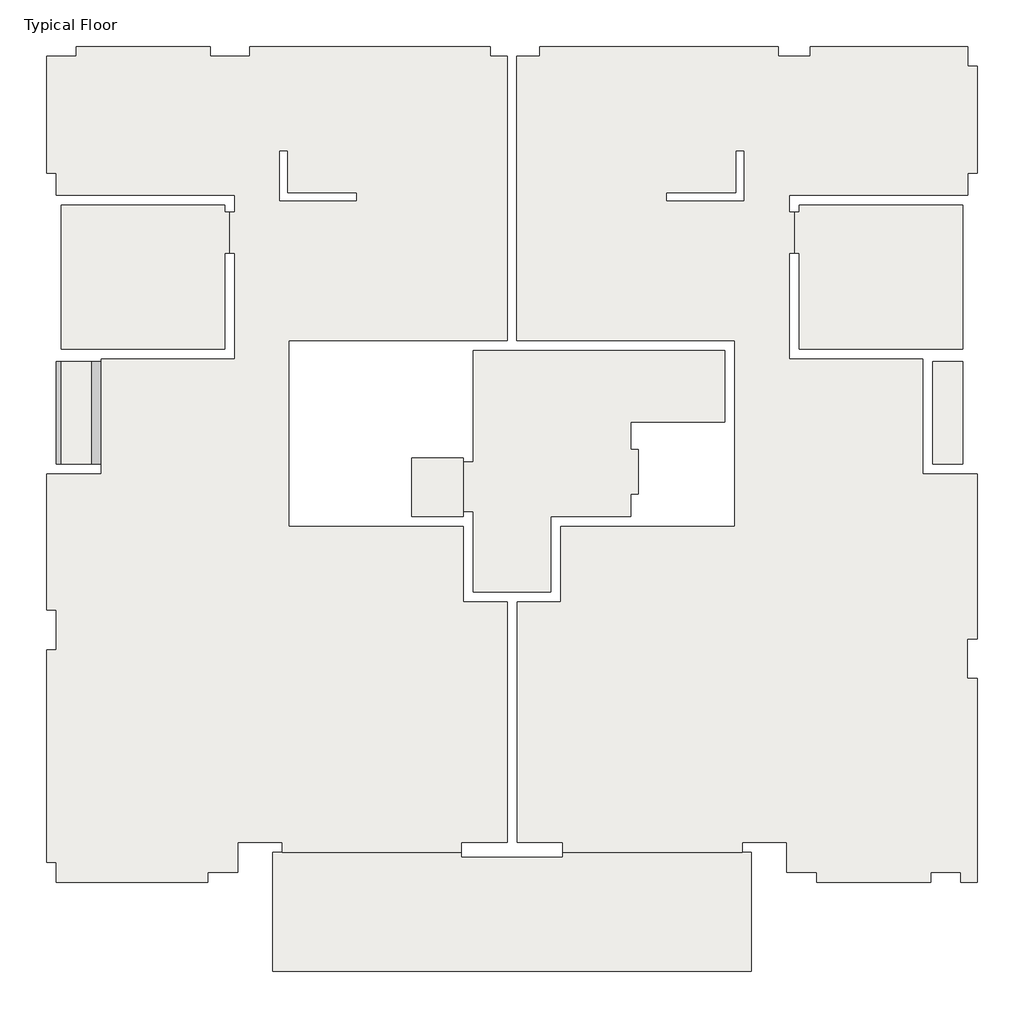
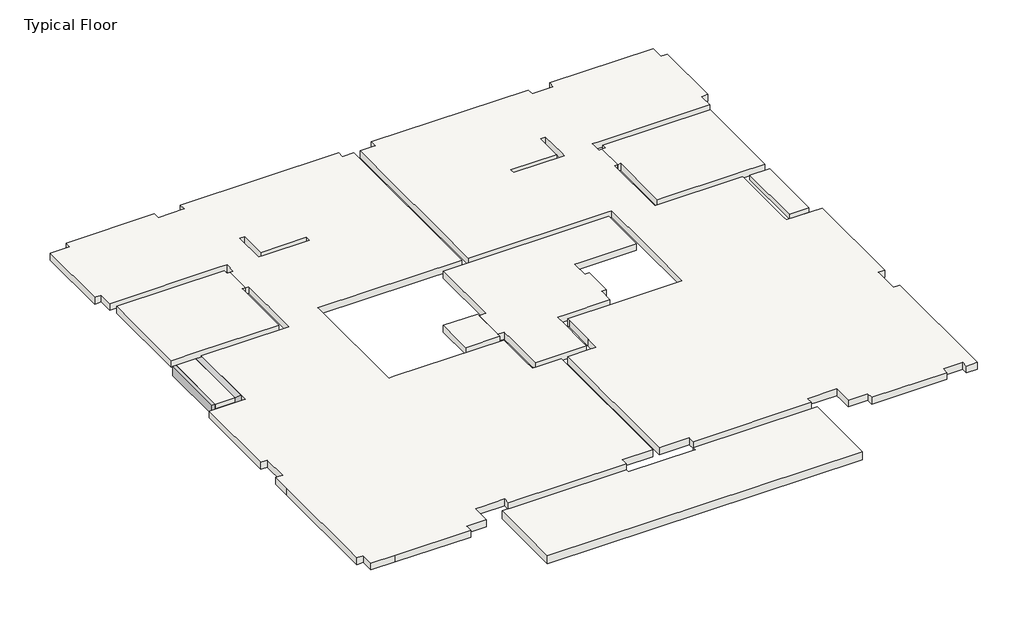
# One storey: 9 slabs, 2 beams.
"""IFC4 building model written with IfcOpenShell, lengths in millimetres."""

from ifc_helpers import new_model, si_unit, frame, origin, place, context, project, spatial, polyline, outline, extrude, faceted_brep, element, save

model = new_model("IFC4")

# Units and contexts
model_context = context("Model", 3, world=origin())
ifc_project = project(units=[si_unit("LENGTHUNIT", "METRE", prefix="MILLI")], contexts=[model_context])

# Site, building, storey
site = spatial("IfcSite", under=ifc_project)
building = spatial("IfcBuilding", under=site)
storey = spatial("IfcBuildingStorey", under=building, Name="Typical Floor", Elevation=3000.0)

# Beams
placement = place(None, origin())
element("IfcBeam", 1, ObjectType="Concrete Rectengular Beam : 10/30", at=placement, inside=storey, context=model_context, shape_type="Brep", body=[
    faceted_brep([(-47605.2156022, 29710.9648817, 3000.0), (-47505.2156022, 29710.9648817, 3000.0), (-47505.2156022, 31780.84273, 3000.0), (-47605.2156022, 31780.84273, 3000.0), (-47605.2156022, 29710.9648817, 2700.0), (-47605.2156022, 31780.84273, 2700.0), (-47505.2156022, 29710.9648817, 2700.0), (-47505.2156022, 31780.84273, 2700.0), (-47505.2156022, 29710.9648817, 2850.0), (-47505.2156022, 31780.84273, 2850.0)], [[[0, 1, 2, 3]], [[4, 0, 3, 5]], [[6, 4, 5, 7]], [[1, 8, 6, 7, 9, 2]], [[1, 0, 4, 6, 8]], [[3, 2, 9, 7, 5]]]),
])
element("IfcBeam", 2, ObjectType="Concrete Rectengular Beam : 20/50", at=placement, inside=storey, context=model_context, shape_type="Brep", body=[
    faceted_brep([(-46905.7952795, 29710.9648817, 3000.0), (-46705.7952795, 29710.9648817, 3000.0), (-46705.7952795, 31780.84273, 3000.0), (-46905.7952795, 31780.84273, 3000.0), (-46905.7952795, 29710.9648817, 2500.0), (-46905.7952795, 29710.9648817, 2850.0), (-46905.7952795, 31780.84273, 2850.0), (-46905.7952795, 31780.84273, 2500.0), (-46705.7952795, 29710.9648817, 2500.0), (-46705.7952795, 31780.84273, 2500.0), (-46705.7952795, 29710.9648817, 2780.0), (-46705.7952795, 31780.84273, 2780.0)], [[[0, 1, 2, 3]], [[4, 5, 0, 3, 6, 7]], [[8, 4, 7, 9]], [[2, 1, 10, 8, 9, 11]], [[1, 0, 5, 4, 8, 10]], [[3, 2, 11, 9, 7, 6]]]),
])

# Slabs
element("IfcSlab", 3, ObjectType="15", at=placement, inside=storey, context=model_context, shape_type="SweptSolid", body=[
    extrude(outline(polyline([(-29340.5251854, 31780.84273), (-29340.5251854, 29710.9648817), (-29944.302346, 29710.9648817), (-29944.302346, 31780.84273), (-29340.5251854, 31780.84273)])), frame((0.0, 0.0, 2850.0), z_axis=(0.0, 0.0, 1.0), x_axis=(1.0, 0.0, 0.0)), (0.0, 0.0, 1.0), 150.0),
])
element("IfcSlab", 4, ObjectType="15", at=placement, inside=storey, context=model_context, shape_type="SweptSolid", body=[
    extrude(outline(polyline([(-47505.2156022, 31780.84273), (-46905.7952795, 31780.84273), (-46905.7952795, 29710.9648817), (-47505.2156022, 29710.9648817), (-47505.2156022, 31780.84273)])), frame((0.0, 0.0, 2850.0), z_axis=(0.0, 0.0, 1.0), x_axis=(1.0, 0.0, 0.0)), (0.0, 0.0, 1.0), 150.0),
])
element("IfcSlab", 5, ObjectType="22", at=placement, inside=storey, context=model_context, shape_type="Brep", body=[
    faceted_brep([(-29045.7952795, 21280.2897882, 2780.0), (-29382.308052, 21280.2897882, 2780.0), (-29382.308052, 21480.2897882, 2780.0), (-29982.308052, 21480.2897882, 2780.0), (-29982.308052, 21280.2897882, 2780.0), (-32286.4740574, 21280.2897882, 2780.0), (-32286.4740574, 21480.2897882, 2780.0), (-32886.4740574, 21480.2897882, 2780.0), (-32886.4740574, 21880.2897882, 2780.0), (-32886.4740574, 22080.2897882, 2780.0), (-33786.4740574, 22080.2897882, 2780.0), (-33786.4740574, 21880.2897882, 2780.0), (-37400.2620822, 21880.2897882, 2780.0), (-37400.2620822, 22079.8085502, 2780.0), (-38324.2014504, 22079.8085502, 2780.0), (-38324.2014504, 26934.5299537, 2780.0), (-37644.7021495, 26934.5299537, 2780.0), (-37444.7021495, 26934.5299537, 2780.0), (-37444.7021495, 27352.982888, 2780.0), (-37444.7021495, 28354.1914622, 2780.0), (-37444.7021495, 28454.7268324, 2780.0), (-35957.8992549, 28454.7268324, 2780.0), (-33933.139307, 28454.7268324, 2780.0), (-33933.139307, 28754.7268324, 2780.0), (-33933.139307, 30454.4375606, 2780.0), (-33933.139307, 32204.3938202, 2780.0), (-34133.139307, 32204.3938202, 2780.0), (-38325.2180585, 32204.3938202, 2780.0), (-38325.2180585, 37931.0505674, 2780.0), (-37865.9301848, 37931.0505674, 2780.0), (-37865.9301848, 38131.0505674, 2780.0), (-33061.2774622, 38131.0505674, 2780.0), (-33061.2774622, 37931.0505674, 2780.0), (-32411.2774622, 37931.0505674, 2780.0), (-32411.2774622, 38131.0505674, 2780.0), (-29244.7343642, 38131.0505674, 2780.0), (-29244.7343642, 37731.0505674, 2780.0), (-29044.7343642, 37731.0505674, 2780.0), (-29044.7343642, 35580.4654108, 2780.0), (-29244.7343642, 35580.4654108, 2780.0), (-29244.7343642, 35129.640202, 2780.0), (-32634.5879334, 35129.640202, 2780.0), (-32834.5879334, 35129.640202, 2780.0), (-32834.5879334, 34793.0831223, 2780.0), (-32734.5879334, 34793.0831223, 2780.0), (-32734.5879334, 33965.4699454, 2780.0), (-32834.5879334, 33965.4699454, 2780.0), (-32834.5879334, 32030.84273, 2780.0), (-32834.5879334, 31830.84273, 2780.0), (-30144.302346, 31830.84273, 2780.0), (-30144.302346, 31780.84273, 2780.0), (-30144.302346, 29710.9648817, 2780.0), (-30144.302346, 29510.9648817, 2780.0), (-29045.7952795, 29510.9648817, 2780.0), (-29045.7952795, 26190.9393744, 2780.0), (-29245.7952795, 26190.9393744, 2780.0), (-29245.7952795, 25390.9393744, 2780.0), (-29045.7952795, 25390.9393744, 2780.0), (-33753.2522949, 36022.8722618, 2780.0), (-33903.2522949, 36022.8722618, 2780.0), (-33903.2522949, 35173.7904306, 2780.0), (-35302.6288773, 35173.7904306, 2780.0), (-35302.6288773, 35023.7904306, 2780.0), (-33753.2522949, 35023.7904306, 2780.0), (-33753.2522949, 35173.7904306, 2780.0), (-29382.308052, 21280.2897882, 3000.0), (-29045.7952795, 21280.2897882, 3000.0), (-29045.7952795, 25390.9393744, 3000.0), (-29245.7952795, 25390.9393744, 3000.0), (-29245.7952795, 26190.9393744, 3000.0), (-29045.7952795, 26190.9393744, 3000.0), (-29045.7952795, 29510.9648817, 3000.0), (-30144.302346, 29510.9648817, 3000.0), (-30144.302346, 29710.9648817, 3000.0), (-30144.302346, 31780.84273, 3000.0), (-30144.302346, 31830.84273, 3000.0), (-32834.5879334, 31830.84273, 3000.0), (-32834.5879334, 32030.84273, 3000.0), (-32834.5879334, 33965.4699454, 3000.0), (-32734.5879334, 33965.4699454, 3000.0), (-32734.5879334, 34793.0831223, 3000.0), (-32834.5879334, 34793.0831223, 3000.0), (-32834.5879334, 35129.640202, 3000.0), (-32634.5879334, 35129.640202, 3000.0), (-29244.7343642, 35129.640202, 3000.0), (-29244.7343642, 35580.4654108, 3000.0), (-29044.7343642, 35580.4654108, 3000.0), (-29044.7343642, 37731.0505674, 3000.0), (-29244.7343642, 37731.0505674, 3000.0), (-29244.7343642, 38131.0505674, 3000.0), (-32411.2774622, 38131.0505674, 3000.0), (-32411.2774622, 37931.0505674, 3000.0), (-33061.2774622, 37931.0505674, 3000.0), (-33061.2774622, 38131.0505674, 3000.0), (-37865.9301848, 38131.0505674, 3000.0), (-37865.9301848, 37931.0505674, 3000.0), (-38325.2180585, 37931.0505674, 3000.0), (-38325.2180585, 32204.3938202, 3000.0), (-34133.139307, 32204.3938202, 3000.0), (-33933.139307, 32204.3938202, 3000.0), (-33933.139307, 30454.4375606, 3000.0), (-33933.139307, 28754.7268324, 3000.0), (-33933.139307, 28454.7268324, 3000.0), (-35957.8992549, 28454.7268324, 3000.0), (-37444.7021495, 28454.7268324, 3000.0), (-37444.7021495, 28354.1914622, 3000.0), (-37444.7021495, 27352.982888, 3000.0), (-37444.7021495, 26934.5299537, 3000.0), (-37644.7021495, 26934.5299537, 3000.0), (-38324.2014504, 26934.5299537, 3000.0), (-38324.2014504, 22079.8085502, 3000.0), (-37400.2620822, 22079.8085502, 3000.0), (-37400.2620822, 21880.2897882, 3000.0), (-33786.4740574, 21880.2897882, 3000.0), (-33786.4740574, 22080.2897882, 3000.0), (-32886.4740574, 22080.2897882, 3000.0), (-32886.4740574, 21880.2897882, 3000.0), (-32886.4740574, 21480.2897882, 3000.0), (-32286.4740574, 21480.2897882, 3000.0), (-32286.4740574, 21280.2897882, 3000.0), (-29982.308052, 21280.2897882, 3000.0), (-29982.308052, 21480.2897882, 3000.0), (-29382.308052, 21480.2897882, 3000.0), (-33903.2522949, 36022.8722618, 3000.0), (-33753.2522949, 36022.8722618, 3000.0), (-33753.2522949, 35173.7904306, 3000.0), (-33753.2522949, 35023.7904306, 3000.0), (-35302.6288773, 35023.7904306, 3000.0), (-35302.6288773, 35173.7904306, 3000.0), (-33903.2522949, 35173.7904306, 3000.0), (-37400.2620822, 21880.2897882, 2800.0)], [[[0, 1, 2, 3, 4, 5, 6, 7, 8, 9, 10, 11, 12, 13, 14, 15, 16, 17, 18, 19, 20, 21, 22, 23, 24, 25, 26, 27, 28, 29, 30, 31, 32, 33, 34, 35, 36, 37, 38, 39, 40, 41, 42, 43, 44, 45, 46, 47, 48, 49, 50, 51, 52, 53, 54, 55, 56, 57], [58, 59, 60, 61, 62, 63, 64]], [[65, 66, 67, 68, 69, 70, 71, 72, 73, 74, 75, 76, 77, 78, 79, 80, 81, 82, 83, 84, 85, 86, 87, 88, 89, 90, 91, 92, 93, 94, 95, 96, 97, 98, 99, 100, 101, 102, 103, 104, 105, 106, 107, 108, 109, 110, 111, 112, 113, 114, 115, 116, 117, 118, 119, 120, 121, 122], [123, 124, 125, 126, 127, 128, 129]], [[1, 0, 66, 65]], [[2, 1, 65, 122]], [[3, 2, 122, 121]], [[4, 3, 121, 120]], [[5, 4, 120, 119]], [[6, 5, 119, 118]], [[7, 6, 118, 117]], [[7, 117, 116, 115, 9, 8]], [[10, 9, 115, 114]], [[11, 10, 114, 113]], [[12, 11, 113, 112, 130]], [[13, 12, 130, 112, 111]], [[14, 13, 111, 110]], [[15, 14, 110, 109]], [[15, 109, 108, 107, 17, 16]], [[18, 17, 107, 106]], [[19, 18, 106, 105]], [[20, 19, 105, 104]], [[20, 104, 103, 102, 22, 21]], [[22, 102, 101, 100, 99, 25, 24, 23]], [[25, 99, 98, 97, 27, 26]], [[28, 27, 97, 96]], [[29, 28, 96, 95]], [[30, 29, 95, 94]], [[31, 30, 94, 93]], [[32, 31, 93, 92]], [[33, 32, 92, 91]], [[34, 33, 91, 90]], [[35, 34, 90, 89]], [[38, 37, 87, 86]], [[39, 38, 86, 85]], [[40, 39, 85, 84]], [[40, 84, 83, 82, 42, 41]], [[43, 42, 82, 81]], [[44, 43, 81, 80]], [[45, 44, 80, 79]], [[46, 45, 79, 78]], [[46, 78, 77, 76, 48, 47]], [[49, 48, 76, 75]], [[49, 75, 74, 73, 72, 52, 51, 50]], [[53, 52, 72, 71]], [[53, 71, 70, 54]], [[0, 57, 67, 66]], [[59, 58, 124, 123]], [[60, 59, 123, 129]], [[61, 60, 129, 128]], [[62, 61, 128, 127]], [[63, 62, 127, 126]], [[63, 126, 125, 124, 58, 64]], [[56, 68, 67, 57]], [[68, 56, 55, 69]], [[69, 55, 54, 70]], [[36, 35, 89, 88]], [[37, 36, 88, 87]]]),
])
element("IfcSlab", 6, ObjectType="22", at=placement, inside=storey, context=model_context, shape_type="Brep", body=[
    faceted_brep([(-44556.7079689, 21280.2897882, 2780.0), (-46866.0948487, 21280.2897882, 2780.0), (-47605.7952795, 21280.2897882, 2780.0), (-47605.7952795, 21680.2897882, 2780.0), (-47805.7952795, 21680.2897882, 2780.0), (-47805.7952795, 25390.9393744, 2780.0), (-47805.7952795, 25968.694731, 2780.0), (-47605.7952795, 25968.694731, 2780.0), (-47605.7952795, 26768.694731, 2780.0), (-47805.7952795, 26768.694731, 2780.0), (-47805.7952795, 29510.9648817, 2780.0), (-46705.7952795, 29510.9648817, 2780.0), (-46705.7952795, 29710.9648817, 2780.0), (-46705.7952795, 31780.84273, 2780.0), (-46705.7952795, 31830.84273, 2780.0), (-44015.8481835, 31830.84273, 2780.0), (-44015.8481835, 32030.84273, 2780.0), (-44015.8481835, 33965.4699454, 2780.0), (-44113.8149674, 33965.4699454, 2780.0), (-44113.8149674, 34793.0831223, 2780.0), (-44015.8481835, 34793.0831223, 2780.0), (-44015.8481835, 35129.640202, 2780.0), (-44215.8481835, 35129.640202, 2780.0), (-47605.7017527, 35129.640202, 2780.0), (-47605.7017527, 35580.4654108, 2780.0), (-47805.7017527, 35580.4654108, 2780.0), (-47805.7017527, 37931.0505674, 2780.0), (-47205.7952795, 37931.0505674, 2780.0), (-47205.7952795, 38131.0505674, 2780.0), (-44508.0144156, 38131.0505674, 2780.0), (-44508.0144156, 37931.0505674, 2780.0), (-43708.0144156, 37931.0505674, 2780.0), (-43708.0144156, 38131.0505674, 2780.0), (-38865.9301848, 38131.0505674, 2780.0), (-38865.9301848, 37931.0505674, 2780.0), (-38525.2180585, 37931.0505674, 2780.0), (-38525.2180585, 32204.3938202, 2780.0), (-42920.5336878, 32204.3938202, 2780.0), (-42920.5336878, 32004.3938202, 2780.0), (-42920.5336878, 28453.6610046, 2780.0), (-42720.5336878, 28453.6610046, 2780.0), (-39404.7173594, 28453.6610046, 2780.0), (-39404.7173594, 28354.1914622, 2780.0), (-39404.7173594, 27352.982888, 2780.0), (-39404.7173594, 26934.5299537, 2780.0), (-39204.7173594, 26934.5299537, 2780.0), (-38524.2014504, 26934.5299537, 2780.0), (-38524.2014504, 22079.8085502, 2780.0), (-39449.2017338, 22079.8085502, 2780.0), (-39449.2017338, 21880.2897882, 2780.0), (-43056.7079689, 21880.2897882, 2780.0), (-43056.7079689, 22080.2897882, 2780.0), (-43756.7079689, 22080.2897882, 2780.0), (-43956.7079689, 22080.2897882, 2780.0), (-43956.7079689, 21480.2897882, 2780.0), (-44556.7079689, 21480.2897882, 2780.0), (-42958.8833647, 36022.8722618, 2780.0), (-43108.8833647, 36022.8722618, 2780.0), (-43108.8833647, 35023.7904306, 2780.0), (-42958.8833647, 35023.7904306, 2780.0), (-41563.7602683, 35023.7904306, 2780.0), (-41563.7602683, 35173.7904306, 2780.0), (-42958.8833647, 35173.7904306, 2780.0), (-46866.0948487, 21280.2897882, 3000.0), (-44556.7079689, 21280.2897882, 3000.0), (-44556.7079689, 21480.2897882, 3000.0), (-43956.7079689, 21480.2897882, 3000.0), (-43956.7079689, 22080.2897882, 3000.0), (-43756.7079689, 22080.2897882, 3000.0), (-43056.7079689, 22080.2897882, 3000.0), (-43056.7079689, 21880.2897882, 3000.0), (-39449.2017338, 21880.2897882, 3000.0), (-39449.2017338, 22079.8085502, 3000.0), (-38524.2014504, 22079.8085502, 3000.0), (-38524.2014504, 26934.5299537, 3000.0), (-39204.7173594, 26934.5299537, 3000.0), (-39404.7173594, 26934.5299537, 3000.0), (-39404.7173594, 27352.982888, 3000.0), (-39404.7173594, 28354.1914622, 3000.0), (-39404.7173594, 28453.6610046, 3000.0), (-42720.5336878, 28453.6610046, 3000.0), (-42920.5336878, 28453.6610046, 3000.0), (-42920.5336878, 32004.3938202, 3000.0), (-42920.5336878, 32204.3938202, 3000.0), (-38525.2180585, 32204.3938202, 3000.0), (-38525.2180585, 37931.0505674, 3000.0), (-38865.9301848, 37931.0505674, 3000.0), (-38865.9301848, 38131.0505674, 3000.0), (-43708.0144156, 38131.0505674, 3000.0), (-43708.0144156, 37931.0505674, 3000.0), (-44508.0144156, 37931.0505674, 3000.0), (-44508.0144156, 38131.0505674, 3000.0), (-47205.7952795, 38131.0505674, 3000.0), (-47205.7952795, 37931.0505674, 3000.0), (-47805.7017527, 37931.0505674, 3000.0), (-47805.7017527, 35580.4654108, 3000.0), (-47605.7017527, 35580.4654108, 3000.0), (-47605.7017527, 35129.640202, 3000.0), (-44215.8481835, 35129.640202, 3000.0), (-44015.8481835, 35129.640202, 3000.0), (-44015.8481835, 34793.0831223, 3000.0), (-44113.8149674, 34793.0831223, 3000.0), (-44113.8149674, 33965.4699454, 3000.0), (-44015.8481835, 33965.4699454, 3000.0), (-44015.8481835, 32030.84273, 3000.0), (-44015.8481835, 31830.84273, 3000.0), (-46705.7952795, 31830.84273, 3000.0), (-46705.7952795, 31780.84273, 3000.0), (-46705.7952795, 29710.9648817, 3000.0), (-46705.7952795, 29510.9648817, 3000.0), (-47805.7952795, 29510.9648817, 3000.0), (-47805.7952795, 26768.694731, 3000.0), (-47605.7952795, 26768.694731, 3000.0), (-47605.7952795, 25968.694731, 3000.0), (-47805.7952795, 25968.694731, 3000.0), (-47805.7952795, 25390.9393744, 3000.0), (-47805.7952795, 21680.2897882, 3000.0), (-47605.7952795, 21680.2897882, 3000.0), (-47605.7952795, 21280.2897882, 3000.0), (-43108.8833647, 36022.8722618, 3000.0), (-42958.8833647, 36022.8722618, 3000.0), (-42958.8833647, 35173.7904306, 3000.0), (-41563.7602683, 35173.7904306, 3000.0), (-41563.7602683, 35023.7904306, 3000.0), (-42958.8833647, 35023.7904306, 3000.0), (-43108.8833647, 35023.7904306, 3000.0), (-39449.2017338, 21880.2897882, 2800.0)], [[[0, 1, 2, 3, 4, 5, 6, 7, 8, 9, 10, 11, 12, 13, 14, 15, 16, 17, 18, 19, 20, 21, 22, 23, 24, 25, 26, 27, 28, 29, 30, 31, 32, 33, 34, 35, 36, 37, 38, 39, 40, 41, 42, 43, 44, 45, 46, 47, 48, 49, 50, 51, 52, 53, 54, 55], [56, 57, 58, 59, 60, 61, 62]], [[63, 64, 65, 66, 67, 68, 69, 70, 71, 72, 73, 74, 75, 76, 77, 78, 79, 80, 81, 82, 83, 84, 85, 86, 87, 88, 89, 90, 91, 92, 93, 94, 95, 96, 97, 98, 99, 100, 101, 102, 103, 104, 105, 106, 107, 108, 109, 110, 111, 112, 113, 114, 115, 116, 117, 118], [119, 120, 121, 122, 123, 124, 125]], [[1, 0, 64, 63]], [[0, 55, 65, 64]], [[55, 54, 66, 65]], [[54, 53, 67, 66]], [[51, 69, 68, 67, 53, 52]], [[51, 50, 70, 69]], [[50, 49, 126, 71, 70]], [[49, 48, 72, 71, 126]], [[48, 47, 73, 72]], [[47, 46, 74, 73]], [[44, 76, 75, 74, 46, 45]], [[44, 43, 77, 76]], [[43, 42, 78, 77]], [[42, 41, 79, 78]], [[39, 81, 80, 79, 41, 40]], [[37, 83, 82, 81, 39, 38]], [[37, 36, 84, 83]], [[36, 35, 85, 84]], [[35, 34, 86, 85]], [[34, 33, 87, 86]], [[33, 32, 88, 87]], [[32, 31, 89, 88]], [[31, 30, 90, 89]], [[30, 29, 91, 90]], [[29, 28, 92, 91]], [[26, 25, 95, 94]], [[25, 24, 96, 95]], [[24, 23, 97, 96]], [[21, 99, 98, 97, 23, 22]], [[21, 20, 100, 99]], [[20, 19, 101, 100]], [[19, 18, 102, 101]], [[18, 17, 103, 102]], [[15, 105, 104, 103, 17, 16]], [[15, 14, 106, 105]], [[11, 109, 108, 107, 106, 14, 13, 12]], [[11, 10, 110, 109]], [[10, 9, 111, 110]], [[5, 4, 116, 115]], [[27, 26, 94, 93]], [[28, 27, 93, 92]], [[57, 56, 120, 119]], [[58, 57, 119, 125]], [[58, 125, 124, 123, 60, 59]], [[61, 60, 123, 122]], [[62, 61, 122, 121]], [[56, 62, 121, 120]], [[2, 1, 63, 118]], [[6, 5, 115, 114]], [[7, 6, 114, 113]], [[8, 7, 113, 112]], [[9, 8, 112, 111]], [[3, 2, 118, 117]], [[4, 3, 117, 116]]]),
])
element("IfcSlab", 7, ObjectType="22", at=placement, inside=storey, context=model_context, shape_type="Brep", body=[
    faceted_brep([(-37644.7021495, 27134.5299537, 2780.0), (-39204.7173594, 27134.5299537, 2780.0), (-39204.7173594, 27352.982888, 2780.0), (-39204.7173594, 28354.1914622, 2780.0), (-39204.7173594, 28754.2406819, 2780.0), (-39404.7173594, 28754.2406819, 2780.0), (-39404.7173594, 29753.278206, 2780.0), (-39204.7173594, 29753.278206, 2780.0), (-39204.7173594, 32004.3938202, 2780.0), (-34133.139307, 32004.3938202, 2780.0), (-34133.139307, 30554.4375606, 2780.0), (-35882.8992549, 30554.4375606, 2780.0), (-36032.8992549, 30554.4375606, 2780.0), (-36032.8992549, 30005.16433, 2780.0), (-35882.8992549, 30005.16433, 2780.0), (-35882.8992549, 29103.4696053, 2780.0), (-36032.8992549, 29103.4696053, 2780.0), (-36032.8992549, 28654.7268324, 2780.0), (-37444.7021495, 28654.7268324, 2780.0), (-37644.7021495, 28654.7268324, 2780.0), (-37644.7021495, 28354.1914622, 2780.0), (-37644.7021495, 27352.982888, 2780.0), (-39204.7173594, 27134.5299537, 3000.0), (-37644.7021495, 27134.5299537, 3000.0), (-37644.7021495, 27352.982888, 3000.0), (-37644.7021495, 28354.1914622, 3000.0), (-37644.7021495, 28654.7268324, 3000.0), (-37444.7021495, 28654.7268324, 3000.0), (-36032.8992549, 28654.7268324, 3000.0), (-36032.8992549, 29103.4696053, 3000.0), (-35882.8992549, 29103.4696053, 3000.0), (-35882.8992549, 30005.16433, 3000.0), (-36032.8992549, 30005.16433, 3000.0), (-36032.8992549, 30554.4375606, 3000.0), (-35882.8992549, 30554.4375606, 3000.0), (-34133.139307, 30554.4375606, 3000.0), (-34133.139307, 32004.3938202, 3000.0), (-39204.7173594, 32004.3938202, 3000.0), (-39204.7173594, 29753.278206, 3000.0), (-39404.7173594, 29753.278206, 3000.0), (-39404.7173594, 28754.2406819, 3000.0), (-39204.7173594, 28754.2406819, 3000.0), (-39204.7173594, 28354.1914622, 3000.0), (-39204.7173594, 27352.982888, 3000.0)], [[[0, 1, 2, 3, 4, 5, 6, 7, 8, 9, 10, 11, 12, 13, 14, 15, 16, 17, 18, 19, 20, 21]], [[22, 23, 24, 25, 26, 27, 28, 29, 30, 31, 32, 33, 34, 35, 36, 37, 38, 39, 40, 41, 42, 43]], [[1, 0, 23, 22]], [[1, 22, 43, 42, 41, 4, 3, 2]], [[5, 4, 41, 40]], [[6, 5, 40, 39]], [[7, 6, 39, 38]], [[8, 7, 38, 37]], [[9, 8, 37, 36]], [[10, 9, 36, 35]], [[10, 35, 34, 33, 12, 11]], [[13, 12, 33, 32]], [[14, 13, 32, 31]], [[15, 14, 31, 30]], [[16, 15, 30, 29]], [[17, 16, 29, 28]], [[17, 28, 27, 26, 19, 18]], [[19, 26, 25, 24, 23, 0, 21, 20]]]),
])
element("IfcSlab", 8, ObjectType="22", at=placement, inside=storey, context=model_context, shape_type="Brep", body=[
    faceted_brep([(-32634.5879334, 34793.0831223, 2780.0), (-32634.5879334, 34929.640202, 2780.0), (-29344.7343642, 34929.640202, 2780.0), (-29344.7343642, 32030.84273, 2780.0), (-32634.5879334, 32030.84273, 2780.0), (-32634.5879334, 33965.4699454, 2780.0), (-32734.5879334, 33965.4699454, 2780.0), (-32734.5879334, 34793.0831223, 2780.0), (-32634.5879334, 34929.640202, 3000.0), (-32634.5879334, 34793.0831223, 3000.0), (-32734.5879334, 34793.0831223, 3000.0), (-32734.5879334, 33965.4699454, 3000.0), (-32634.5879334, 33965.4699454, 3000.0), (-32634.5879334, 32030.84273, 3000.0), (-30144.302346, 32030.84273, 3000.0), (-29344.7343642, 32030.84273, 3000.0), (-29344.7343642, 34929.640202, 3000.0)], [[[0, 1, 2, 3, 4, 5, 6, 7]], [[8, 9, 10, 11, 12, 13, 14, 15, 16]], [[1, 0, 9, 8]], [[2, 1, 8, 16]], [[3, 2, 16, 15]], [[4, 3, 15, 14, 13]], [[5, 4, 13, 12]], [[6, 5, 12, 11]], [[7, 6, 11, 10]], [[0, 7, 10, 9]]]),
])
element("IfcSlab", 9, ObjectType="22", at=placement, inside=storey, context=model_context, shape_type="Brep", body=[
    faceted_brep([(-44215.8481835, 34929.640202, 2780.0), (-44215.8481835, 34793.0831223, 2780.0), (-44113.8149674, 34793.0831223, 2780.0), (-44113.8149674, 33965.4699454, 2780.0), (-44215.8481835, 33965.4699454, 2780.0), (-44215.8481835, 32030.84273, 2780.0), (-47505.7017527, 32030.84273, 2780.0), (-47505.7017527, 34929.640202, 2780.0), (-44215.8481835, 34793.0831223, 3000.0), (-44215.8481835, 34929.640202, 3000.0), (-47505.7017527, 34929.640202, 3000.0), (-47505.7017527, 32030.84273, 3000.0), (-46705.7952795, 32030.84273, 3000.0), (-44215.8481835, 32030.84273, 3000.0), (-44215.8481835, 33965.4699454, 3000.0), (-44113.8149674, 33965.4699454, 3000.0), (-44113.8149674, 34793.0831223, 3000.0)], [[[0, 1, 2, 3, 4, 5, 6, 7]], [[8, 9, 10, 11, 12, 13, 14, 15, 16]], [[1, 0, 9, 8]], [[2, 1, 8, 16]], [[3, 2, 16, 15]], [[4, 3, 15, 14]], [[4, 14, 13, 5]], [[10, 7, 6, 11]], [[0, 7, 10, 9]], [[5, 13, 12, 11, 6]]]),
])
element("IfcSlab", 10, ObjectType="22", at=placement, inside=storey, context=model_context, shape_type="Brep", body=[
    faceted_brep([(-40450.3660009, 29837.9491617, 2780.0), (-39404.7173594, 29837.9491617, 2780.0), (-39404.7173594, 29753.278206, 2780.0), (-39404.7173594, 28754.2406819, 2780.0), (-39404.7173594, 28653.6610046, 2780.0), (-40450.3660009, 28653.6610046, 2780.0), (-39404.7173594, 29837.9491617, 3000.0), (-40450.3660009, 29837.9491617, 3000.0), (-40450.3660009, 28653.6610046, 3000.0), (-39404.7173594, 28653.6610046, 3000.0), (-39404.7173594, 28754.2406819, 3000.0), (-39404.7173594, 29753.278206, 3000.0)], [[[0, 1, 2, 3, 4, 5]], [[6, 7, 8, 9, 10, 11]], [[1, 0, 7, 6]], [[3, 2, 1, 6, 11, 10]], [[3, 10, 9, 4]], [[7, 0, 5, 8]], [[5, 4, 9, 8]]]),
])
element("IfcSlab", 11, ObjectType="26", at=placement, inside=storey, context=model_context, shape_type="Brep", body=[
    faceted_brep([(-39449.2017338, 21880.2897882, 2540.0), (-39449.2017338, 21779.8085502, 2540.0), (-37400.2620822, 21779.8085502, 2540.0), (-37400.2620822, 21880.2897882, 2540.0), (-33605.0891993, 21880.2897882, 2540.0), (-33605.0891993, 19481.1095176, 2540.0), (-43243.3137014, 19481.1095176, 2540.0), (-43243.3137014, 21880.2897882, 2540.0), (-39449.2017338, 21779.8085502, 2800.0), (-39449.2017338, 21880.2897882, 2800.0), (-43056.7079689, 21880.2897882, 2800.0), (-43243.3137014, 21880.2897882, 2800.0), (-43243.3137014, 19481.1095176, 2800.0), (-33605.0891993, 19481.1095176, 2800.0), (-33605.0891993, 21880.2897882, 2800.0), (-33786.4740574, 21880.2897882, 2800.0), (-37400.2620822, 21880.2897882, 2800.0), (-37400.2620822, 21779.8085502, 2800.0), (-39449.2017338, 21880.2897882, 2780.0), (-37400.2620822, 21880.2897882, 2780.0), (-33605.0891993, 21880.2897882, 2600.0), (-33605.0891993, 19481.1095176, 2600.0), (-43243.3137014, 19481.1095176, 2600.0), (-43243.3137014, 21880.2897882, 2600.0)], [[[0, 1, 2, 3, 4, 5, 6, 7]], [[8, 9, 10, 11, 12, 13, 14, 15, 16, 17]], [[1, 0, 18, 9, 8]], [[2, 1, 8, 17]], [[3, 2, 17, 16, 19]], [[4, 3, 19, 16, 15, 14, 20]], [[5, 4, 20, 14, 13, 21]], [[6, 5, 21, 13, 12, 22]], [[7, 6, 22, 12, 11, 23]], [[0, 7, 23, 11, 10, 9, 18]]]),
])

save(model, "model.ifc")

# Revit data of these elements
# Type "Concrete Rectengular Beam : 10/30"
#   Length [instance default] = 152.4 cm
#   b = 10 cm
#   h = 30 cm
#   Structural Material [instance default] = Concrete
#   Assembly Code = ""
# Type "Concrete Rectengular Beam : 20/50"
#   Length [instance default] = 152.4 cm
#   b = 20 cm
#   h = 50 cm
#   Structural Material [instance default] = Concrete
#   Assembly Code = ""
# Type "15"
#   Function = 0
#   Layers, outside or top first: 15 cm "Concrete" (function 1)
# Type "22"
#   Function = 0
#   Layers, outside or top first: 22 cm "Concrete" (function 1)
# Type "26"
#   Function = 0
#   Layers, outside or top first: 26 cm "Concrete" (function 1)
# Element 1 (IfcBeam, "Concrete Rectengular Beam : 10/30")
#   Comments = ""
#   Mark = "B2"
#   SOFiSTiK_AMG_Comments = "Too Narrow Beam /"
#   SOFiSTiK_AMG_Scheduled = yes
#   SOFiSTiK_AMG_Adjusted = yes
#   Structural Material = Concrete
#   Phase Created = New Construction
#   Materials on its faces: "Concrete"
# Element 2 (IfcBeam, "Concrete Rectengular Beam : 20/50")
#   Comments = ""
#   Mark = "B6"
#   SOFiSTiK_AMG_Comments = ""
#   SOFiSTiK_AMG_Scheduled = yes
#   SOFiSTiK_AMG_Adjusted = yes
#   Structural Material = Concrete
#   Phase Created = New Construction
#   Materials on its faces: "Concrete"
# Element 3 (IfcSlab, "15")
#   Mark = "S7"
#   SOFiSTiK_AMG_Comments = ""
#   Height Offset From Level = 0 cm
#   built-in parameter 1001954 = 1
#   SOFiSTiK_AMG_Scheduled = yes
#   SOFiSTiK_AMG_Adjusted = yes
#   Phase Created = New Construction
#   Materials on its faces: "Concrete"
# Element 4 (IfcSlab, "15")
#   Mark = "S8"
#   SOFiSTiK_AMG_Comments = ""
#   built-in parameter 1001955 = 3.14159 (stored number, unit not read)
#   Height Offset From Level = 0 cm
#   built-in parameter 1001954 = 1
#   SOFiSTiK_AMG_Scheduled = yes
#   SOFiSTiK_AMG_Adjusted = yes
#   Phase Created = New Construction
#   Materials on its faces: "Concrete"
# Element 5 (IfcSlab, "22")
#   Mark = "S1"
#   SOFiSTiK_AMG_Comments = ""
#   built-in parameter 1001955 = -1.5708 (stored number, unit not read)
#   Height Offset From Level = 0 cm
#   built-in parameter 1001954 = 1
#   SOFiSTiK_AMG_Scheduled = yes
#   SOFiSTiK_AMG_Adjusted = no
#   Phase Created = New Construction
#   Materials on its faces: "Concrete"
# Element 6 (IfcSlab, "22")
#   Mark = "S2"
#   SOFiSTiK_AMG_Comments = ""
#   built-in parameter 1001955 = -1.5708 (stored number, unit not read)
#   Height Offset From Level = 0 cm
#   built-in parameter 1001954 = 1
#   SOFiSTiK_AMG_Scheduled = yes
#   SOFiSTiK_AMG_Adjusted = yes
#   Phase Created = New Construction
#   Materials on its faces: "Concrete"
# Element 7 (IfcSlab, "22")
#   Mark = "S3"
#   SOFiSTiK_AMG_Comments = ""
#   built-in parameter 1001955 = -1.5708 (stored number, unit not read)
#   Height Offset From Level = 0 cm
#   built-in parameter 1001954 = 1
#   SOFiSTiK_AMG_Scheduled = yes
#   SOFiSTiK_AMG_Adjusted = yes
#   Phase Created = New Construction
#   Materials on its faces: "Concrete"
# Element 8 (IfcSlab, "22")
#   Mark = "S4"
#   SOFiSTiK_AMG_Comments = ""
#   Height Offset From Level = 0 cm
#   built-in parameter 1001954 = 1
#   SOFiSTiK_AMG_Scheduled = yes
#   SOFiSTiK_AMG_Adjusted = yes
#   Phase Created = New Construction
#   Materials on its faces: "Concrete"
# Element 9 (IfcSlab, "22")
#   Mark = "S5"
#   SOFiSTiK_AMG_Comments = ""
#   Height Offset From Level = 0 cm
#   built-in parameter 1001954 = 1
#   SOFiSTiK_AMG_Scheduled = yes
#   SOFiSTiK_AMG_Adjusted = yes
#   Phase Created = New Construction
#   Materials on its faces: "Concrete"
# Element 10 (IfcSlab, "22")
#   Mark = "S6"
#   SOFiSTiK_AMG_Comments = ""
#   built-in parameter 1001955 = 3.14159 (stored number, unit not read)
#   Height Offset From Level = 0 cm
#   built-in parameter 1001954 = 1
#   SOFiSTiK_AMG_Scheduled = yes
#   SOFiSTiK_AMG_Adjusted = yes
#   Phase Created = New Construction
#   Materials on its faces: "Concrete"
# Element 11 (IfcSlab, "26")
#   Mark = "S10"
#   SOFiSTiK_AMG_Comments = ""
#   Height Offset From Level = -20 cm
#   built-in parameter 1001954 = 1
#   SOFiSTiK_AMG_Scheduled = yes
#   SOFiSTiK_AMG_Adjusted = yes
#   Phase Created = New Construction
#   Materials on its faces: "Concrete"
# Materials
#   "Concrete": class "Concrete", colour RGB 192 192 192, transparency 0, Keynote = "01000", Description = "Cast-in-place concrete", Cost = 0
